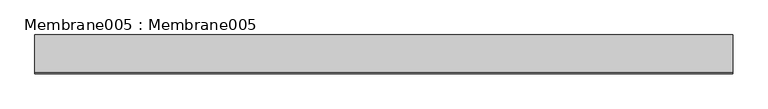
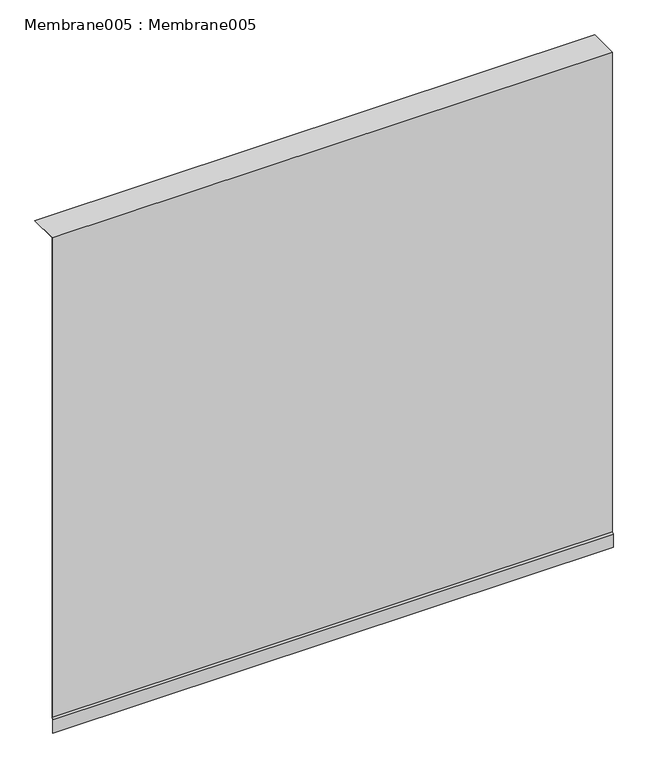
"""IFC4 building model written with IfcOpenShell, lengths in millimetres: proxy geometry, Membrane005 : Membrane005."""

import ifcopenshell
import ifcopenshell.guid

model = None  # the IFC model being written
_history = None  # IfcOwnerHistory: only IFC2X3 demands one
_inside = {}  # id of a spatial element -> (the spatial element, [elements in it])
_under = {}  # id of a project, library or spatial element -> (it, [spatial elements below it])
_declared = {}  # id of a project -> (the project, [libraries it declares])
_typed = {}  # id of a type object -> (the type object, [elements of that type])
_made_of = {}  # id of a material, layer set ... -> (it, [elements and type objects made of it])


def new_model(schema):
    """Start an empty IFC model of exactly this schema.

    Asked for "IFC4X3", IfcOpenShell would pick the latest addendum, in which some entities
    have other attributes; the version numbers below select the first issue.
    IFC2X3 requires an IfcOwnerHistory on every rooted entity: one is made here for all.
    """
    global model, _history
    if schema == "IFC4X3":
        model = ifcopenshell.file(schema_version=(4, 3, 0, 0))
    else:
        model = ifcopenshell.file(schema=schema)
    _inside.clear()
    _under.clear()
    _declared.clear()
    _typed.clear()
    _made_of.clear()
    _history = None
    if model.schema == "IFC2X3":
        org = make("IfcOrganization", Name="unknown")
        user = make(
            "IfcPersonAndOrganization",
            ThePerson=make("IfcPerson", FamilyName="unknown"),
            TheOrganization=org,
        )
        app = make(
            "IfcApplication",
            ApplicationDeveloper=org,
            Version="unknown",
            ApplicationFullName="unknown",
            ApplicationIdentifier="unknown",
        )
        _history = make(
            "IfcOwnerHistory",
            OwningUser=user,
            OwningApplication=app,
            ChangeAction="ADDED",
            CreationDate=0,
        )
    return model


def make(cls, **values):
    """One entity of the class cls with the attributes given. An attribute that is None is left unset."""
    return model.create_entity(
        cls, **{name: value for name, value in values.items() if value is not None}
    )


def rooted(cls, **values):
    """An entity with a GlobalId (a new one), such as an element, a storey or a relation."""
    return make(cls, GlobalId=ifcopenshell.guid.new(), OwnerHistory=_history, **values)


def si_unit(unit_type, name, prefix=None):
    """IfcSIUnit, for example si_unit("LENGTHUNIT", "METRE", prefix="MILLI")."""
    return make("IfcSIUnit", UnitType=unit_type, Prefix=prefix, Name=name)


def assignment(units):
    """IfcUnitAssignment: the units of a project."""
    return None if units is None else make("IfcUnitAssignment", Units=units)


def point(xyz):
    """IfcCartesianPoint."""
    return None if xyz is None else make("IfcCartesianPoint", Coordinates=xyz)


def direction(xyz):
    """IfcDirection."""
    return None if xyz is None else make("IfcDirection", DirectionRatios=xyz)


def frame(location, z_axis=None, x_axis=None):
    """IfcAxis2Placement3D, a coordinate frame: its origin and axes. An axis left out is left unset."""
    return make(
        "IfcAxis2Placement3D",
        Location=point(location),
        Axis=direction(z_axis),
        RefDirection=direction(x_axis),
    )


def origin():
    """The frame at (0, 0, 0) with its axes left unset."""
    return frame((0.0, 0.0, 0.0))


def place(relative_to, where):
    """IfcLocalPlacement: puts the frame where relative to a parent placement (None: the world)."""
    return make(
        "IfcLocalPlacement", PlacementRelTo=relative_to, RelativePlacement=where
    )


def context(
    kind, dimensions, precision=None, world=None, true_north=None, identifier=None
):
    """IfcGeometricRepresentationContext, for example the 3D "Model" context."""
    return make(
        "IfcGeometricRepresentationContext",
        ContextIdentifier=identifier,
        ContextType=kind,
        CoordinateSpaceDimension=dimensions,
        Precision=precision,
        WorldCoordinateSystem=world,
        TrueNorth=true_north,
    )


def project(units=None, contexts=None):
    """IfcProject with its units and contexts."""
    return rooted(
        "IfcProject",
        Name="project",
        RepresentationContexts=contexts,
        UnitsInContext=assignment(units),
    )


def spatial(cls, under=None, at=None, **own):
    """A site, building, storey or space (cls), placed at a placement, below another one or the project."""
    s = rooted(cls, ObjectPlacement=at, **own)
    if under is not None:
        _under.setdefault(under.id(), (under, []))[1].append(s)
    return s


def polyline(points):
    """IfcPolyline through the points."""
    return make("IfcPolyline", Points=[point(p) for p in points])


def outline(outer, holes=None, kind="AREA"):
    """IfcArbitraryClosedProfileDef: a profile drawn as a closed curve; with holes, ...WithVoids."""
    if holes is None:
        return make("IfcArbitraryClosedProfileDef", ProfileType=kind, OuterCurve=outer)
    return make(
        "IfcArbitraryProfileDefWithVoids",
        ProfileType=kind,
        OuterCurve=outer,
        InnerCurves=holes,
    )


def extrude(swept, where, along, depth):
    """IfcExtrudedAreaSolid: the profile swept, set in the frame where, extruded along a direction by depth."""
    return make(
        "IfcExtrudedAreaSolid",
        SweptArea=swept,
        Position=where,
        ExtrudedDirection=direction(along),
        Depth=depth,
    )


def shape(context_of_items, identifier, shape_type, items):
    """IfcShapeRepresentation: the items that make up one representation, for example the "Body"."""
    return make(
        "IfcShapeRepresentation",
        ContextOfItems=context_of_items,
        RepresentationIdentifier=identifier,
        RepresentationType=shape_type,
        Items=items,
    )


def source(mapping_origin, context_of_items, identifier, shape_type, items):
    """IfcRepresentationMap: a shape defined once, which mapped items show again and again."""
    return make(
        "IfcRepresentationMap",
        MappingOrigin=mapping_origin,
        MappedRepresentation=shape(context_of_items, identifier, shape_type, items),
    )


def transform(
    local_origin,
    x_axis=None,
    y_axis=None,
    z_axis=None,
    scale=None,
    scale2=None,
    scale3=None,
    uniform=True,
):
    """IfcCartesianTransformationOperator3D, or its non-uniform kind. x_axis, y_axis, z_axis: its Axis1, 2, 3."""
    if uniform:
        return make(
            "IfcCartesianTransformationOperator3D",
            Axis1=direction(x_axis),
            Axis2=direction(y_axis),
            LocalOrigin=point(local_origin),
            Scale=scale,
            Axis3=direction(z_axis),
        )
    return make(
        "IfcCartesianTransformationOperator3DnonUniform",
        Axis1=direction(x_axis),
        Axis2=direction(y_axis),
        LocalOrigin=point(local_origin),
        Scale=scale,
        Axis3=direction(z_axis),
        Scale2=scale2,
        Scale3=scale3,
    )


def mapped(mapping_source, mapping_target):
    """IfcMappedItem: shows the shape of a source again, moved by a transform."""
    return make(
        "IfcMappedItem", MappingSource=mapping_source, MappingTarget=mapping_target
    )


def made_of(thing, what):
    """Note that an element or type object is made of a material, layer set ...; save() writes the relation."""
    if what is not None:
        _made_of.setdefault(what.id(), (what, []))[1].append(thing)
    return thing


def element(
    cls,
    number,
    at=None,
    inside=None,
    cuts=None,
    type_object=None,
    material=None,
    context=None,
    identifier="Body",
    shape_type=None,
    held_by="IfcProductDefinitionShape",
    body=None,
    shapes=None,
    **own,
):
    """One element of the class cls, such as IfcWall. Its Tag is "e" and its number.

    at: its placement. inside: the storey or other place that contains it. cuts: it is an
    opening in that element (IfcRelVoidsElement). A single representation is given by context,
    identifier, shape_type and body (its items); several are given by shapes. held_by: the class
    of the entity that holds the representations. save() writes the other relations.
    """
    e = rooted(cls, Tag="e%d" % number, ObjectPlacement=at, **own)
    if body is not None:
        shapes = [shape(context, identifier, shape_type, body)]
    if shapes is not None:
        e.Representation = make(held_by, Representations=shapes)
    if inside is not None:
        _inside.setdefault(inside.id(), (inside, []))[1].append(e)
    if cuts is not None:
        rooted(
            "IfcRelVoidsElement", RelatingBuildingElement=cuts, RelatedOpeningElement=e
        )
    if type_object is not None:
        _typed.setdefault(type_object.id(), (type_object, []))[1].append(e)
    return made_of(e, material)


def aggregate(whole, parts):
    """IfcRelAggregates: a whole, such as a stair, and the parts it consists of."""
    return rooted("IfcRelAggregates", RelatingObject=whole, RelatedObjects=parts)


def save(model, path):
    """Write the relations noted so far, then the file.

    IfcRelAggregates (storeys below a building ...), IfcRelContainedInSpatialStructure (elements
    in a storey), IfcRelDefinesByType, IfcRelAssociatesMaterial and IfcRelDeclares: one each for
    every whole, place, type object, material and project.
    """
    for whole, parts in _under.values():
        aggregate(whole, parts)
    for where, things in _inside.values():
        rooted(
            "IfcRelContainedInSpatialStructure",
            RelatedElements=things,
            RelatingStructure=where,
        )
    for kind, things in _typed.values():
        rooted("IfcRelDefinesByType", RelatedObjects=things, RelatingType=kind)
    for what, things in _made_of.values():
        rooted("IfcRelAssociatesMaterial", RelatedObjects=things, RelatingMaterial=what)
    for by, libraries in _declared.values():
        rooted("IfcRelDeclares", RelatingContext=by, RelatedDefinitions=libraries)
    model.write(path)


def membrane005_membrane005_4d7ae10d(model_context):
    return source(origin(), model_context, "Body", "SweptSolid", [
        extrude(outline(polyline([(-4662.0876539, 36597.8828125), (-4662.0876539, 36548.0898437), (-4663.5876539, 36548.0898437), (-4663.5876539, 36598.2944693), (-4659.4279428, 36605.3022818), (-4659.4279428, 38413.7101562), (-4552.1284743, 38413.7101562), (-4552.1284743, 38412.2101562), (-4657.9279428, 38412.2101562), (-4657.9279428, 36604.890625), (-4662.0876539, 36597.8828125)])), frame((12383.0178845, 0.0, 0.0), z_axis=(1.0, 0.0, 0.0), x_axis=(0.0, 1.0, 0.0)), (0.0, 0.0, 1.0), 2000.0),
    ])


if __name__ == "__main__":
    model = new_model("IFC4")
    model_context = context("Model", 3, world=origin())
    ifc_project = project(units=[si_unit("LENGTHUNIT", "METRE", prefix="MILLI")], contexts=[model_context])
    site = spatial("IfcSite", under=ifc_project)
    building = spatial("IfcBuilding", under=site)
    placement = place(None, origin())
    membrane005_membrane005_shape = membrane005_membrane005_4d7ae10d(model_context)
    element("IfcBuildingElementProxy", 1, Name="Membrane005 : Membrane005", ObjectType="Membrane005 : Membrane005", at=placement, inside=building, context=model_context, shape_type="MappedRepresentation", body=[
        mapped(membrane005_membrane005_shape, transform((0.0, 0.0, 0.0), x_axis=(1.0, 0.0, 0.0), y_axis=(0.0, 1.0, 0.0), z_axis=(0.0, 0.0, 1.0))),
    ])
    save(model, "model.ifc")

# Revit data of these elements
# Type "Membrane005 : Membrane005"
#   NameOverride = "Membrane005"
# Element 1 (IfcBuildingElementProxy, "Membrane005 : Membrane005")
#   Materials on its faces: "2 LAYERS NO. 30 ASTM D226 ASPHALT SATURATED ORGANIC FELT"
# Materials
#   "2 LAYERS NO. 30 ASTM D226 ASPHALT SATURATED ORGANIC FELT": class "Unassigned", colour RGB 46 171 0, transparency 0
